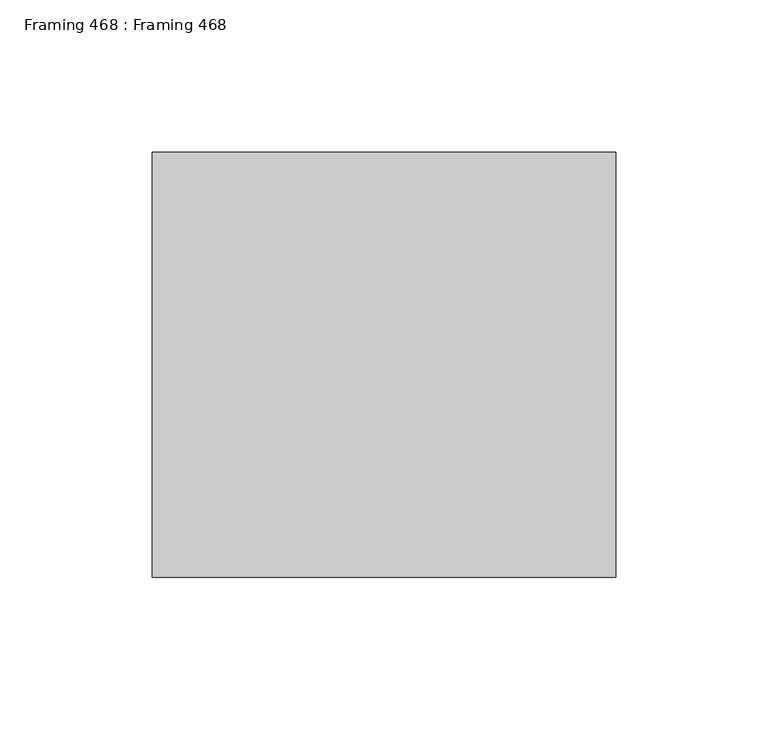
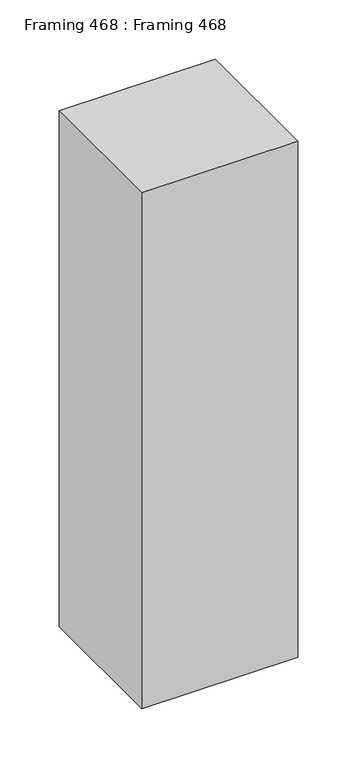
"""IFC4 building model written with IfcOpenShell, lengths in millimetres: proxy geometry, Framing 468 : Framing 468."""

from ifc_helpers import new_model, si_unit, frame, origin, place, context, project, spatial, polyline, outline, extrude, source, transform, mapped, element, save


def framing_468_framing_468_917e6005(model_context):
    return source(origin(), model_context, "Body", "SweptSolid", [
        extrude(outline(polyline([(5541.8883192, 10278.0250834), (5541.8883192, 10417.7250834), (5694.2883192, 10417.7250834), (5694.2883192, 10278.0250834), (5541.8883192, 10278.0250834)])), frame((0.0, 0.0, 40138.0976562), z_axis=(0.0, 0.0, 1.0), x_axis=(1.0, 0.0, 0.0)), (0.0, 0.0, 1.0), 533.4),
    ])


if __name__ == "__main__":
    model = new_model("IFC4")
    model_context = context("Model", 3, world=origin())
    ifc_project = project(units=[si_unit("LENGTHUNIT", "METRE", prefix="MILLI")], contexts=[model_context])
    site = spatial("IfcSite", under=ifc_project)
    building = spatial("IfcBuilding", under=site)
    placement = place(None, origin())
    framing_468_framing_468_shape = framing_468_framing_468_917e6005(model_context)
    element("IfcBuildingElementProxy", 1, Name="Framing 468 : Framing 468", ObjectType="Framing 468 : Framing 468", at=placement, inside=building, context=model_context, shape_type="MappedRepresentation", body=[
        mapped(framing_468_framing_468_shape, transform((0.0, 0.0, 0.0), x_axis=(1.0, 0.0, 0.0), y_axis=(0.0, 1.0, 0.0), z_axis=(0.0, 0.0, 1.0))),
    ])
    save(model, "model.ifc")

# Revit data of these elements
# Type "Framing 468 : Framing 468"
#   NameOverride = "Framing"
# Element 1 (IfcBuildingElementProxy, "Framing 468 : Framing 468")
#   Materials on its faces: "WOOD FRAMING (SEE STRUCT DWGS)"
# Materials
#   "WOOD FRAMING (SEE STRUCT DWGS)": class "Unassigned", colour RGB 224 188 168, transparency 0, Cost = 0
